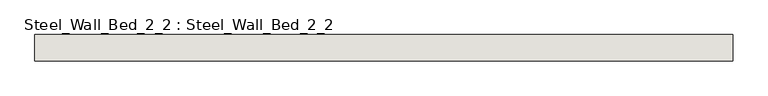
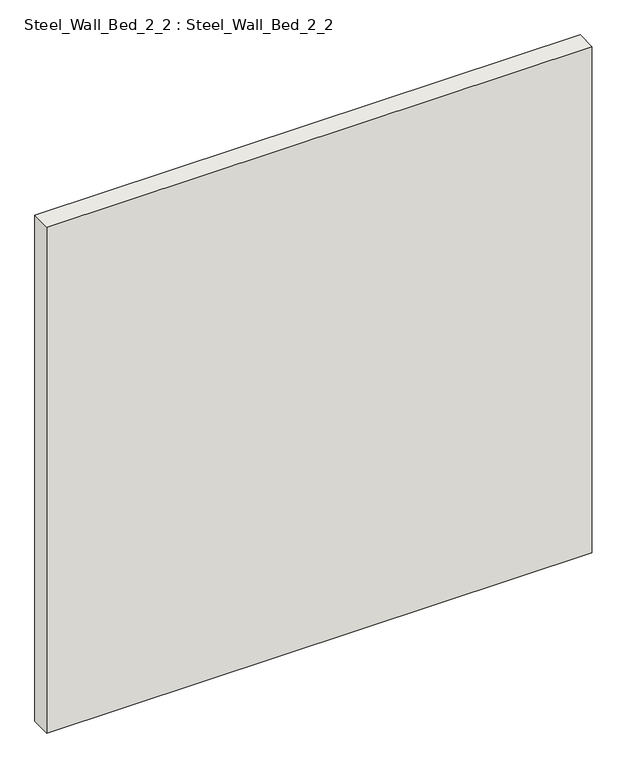
"""IFC4 building model written with IfcOpenShell, lengths in millimetres: wall geometry, Steel_Wall_Bed_2_2 : Steel_Wall_Bed_2_2."""

from ifc_helpers import new_model, si_unit, frame, origin, place, context, project, spatial, polyline, outline, extrude, source, transform, mapped, element, save


def steel_wall_bed_2_2_steel_wall_bed_2_2_f5710ee6(model_context):
    return source(origin(), model_context, "Body", "SweptSolid", [
        extrude(outline(polyline([(4265.0, 8795.0), (1615.0, 8795.0), (1615.0, 8895.0), (4265.0, 8895.0), (4265.0, 8795.0)])), frame((0.0, 0.0, 250.0), z_axis=(0.0, 0.0, 1.0), x_axis=(1.0, 0.0, 0.0)), (0.0, 0.0, 1.0), 2600.0),
    ])


if __name__ == "__main__":
    model = new_model("IFC4")
    model_context = context("Model", 3, world=origin())
    ifc_project = project(units=[si_unit("LENGTHUNIT", "METRE", prefix="MILLI")], contexts=[model_context])
    site = spatial("IfcSite", under=ifc_project)
    building = spatial("IfcBuilding", under=site)
    placement = place(None, origin())
    steel_wall_bed_2_2_steel_wall_bed_2_2_shape = steel_wall_bed_2_2_steel_wall_bed_2_2_f5710ee6(model_context)
    element("IfcWall", 1, ObjectType="Steel_Wall_Bed_2_2 : Steel_Wall_Bed_2_2", at=placement, inside=building, context=model_context, shape_type="MappedRepresentation", body=[
        mapped(steel_wall_bed_2_2_steel_wall_bed_2_2_shape, transform((0.0, 0.0, 0.0), x_axis=(1.0, 0.0, 0.0), y_axis=(0.0, 1.0, 0.0), z_axis=(0.0, 0.0, 1.0))),
    ])
    save(model, "model.ifc")

# Revit data of these elements
# Type "Steel_Wall_Bed_2_2 : Steel_Wall_Bed_2_2"
#   NameOverride = "Steel_Wall_Bed_2_2"
# Element 1 (IfcWall, "Steel_Wall_Bed_2_2 : Steel_Wall_Bed_2_2")
#   Materials on its faces: "IfcSurfaceStyle #33"
# Materials
#   "IfcSurfaceStyle #33": class "Unassigned", colour RGB 214 214 214, transparency 0
